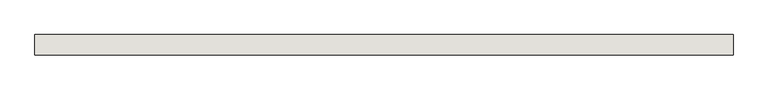
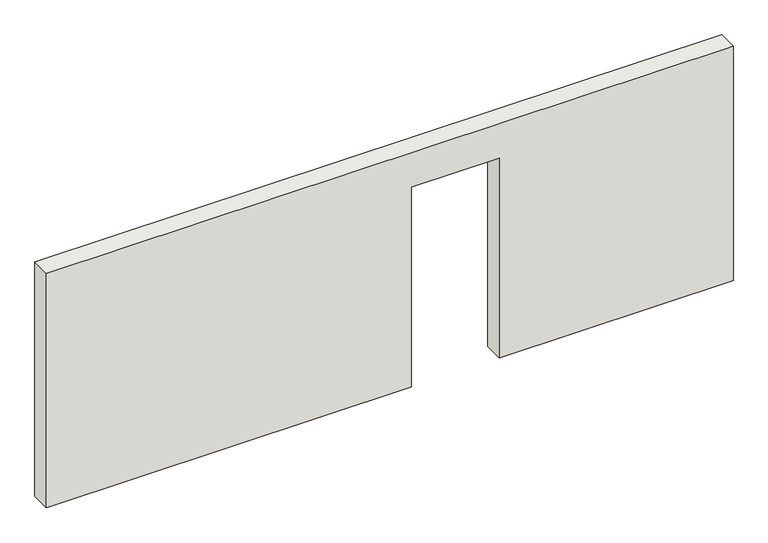
"""IFC4 building model written with IfcOpenShell, lengths in millimetres: wall geometry, Holzwand."""

from ifc_helpers import new_model, si_unit, frame, origin, place, context, project, spatial, polyline, outline, extrude, source, transform, mapped, element, save


def wall_de2372fb(model_context):
    return source(origin(), model_context, "Body", "SweptSolid", [
        extrude(outline(polyline([(0.0, 3680.0), (2135.0, 3680.0), (2135.0, 4565.0), (0.0, 4565.0), (0.0, 6925.0), (2500.0, 6925.0), (2500.0, 0.0), (0.0, 0.0), (0.0, 3680.0)])), frame((0.0, 0.0, 0.0), z_axis=(0.0, 1.0, 0.0), x_axis=(0.0, 0.0, 1.0)), (0.0, 0.0, 1.0), 200.0),
    ])


if __name__ == "__main__":
    model = new_model("IFC4")
    model_context = context("Model", 3, world=origin())
    ifc_project = project(units=[si_unit("LENGTHUNIT", "METRE", prefix="MILLI")], contexts=[model_context])
    site = spatial("IfcSite", under=ifc_project)
    building = spatial("IfcBuilding", under=site)
    placement = place(None, origin())
    wall_shape = wall_de2372fb(model_context)
    element("IfcWall", 1, ObjectType="Holzwand", at=placement, inside=building, context=model_context, shape_type="MappedRepresentation", body=[
        mapped(wall_shape, transform((0.0, 0.0, 0.0), x_axis=(1.0, 0.0, 0.0), y_axis=(0.0, 1.0, 0.0), z_axis=(0.0, 0.0, 1.0))),
    ])
    save(model, "model.ifc")

# Revit data of these elements
# Element 1 (IfcWall, "Holzwand")
#   Materials on its faces: "holzschalung"
# Materials
#   "holzschalung": class "Unassigned", colour RGB 128 128 128, transparency 0
